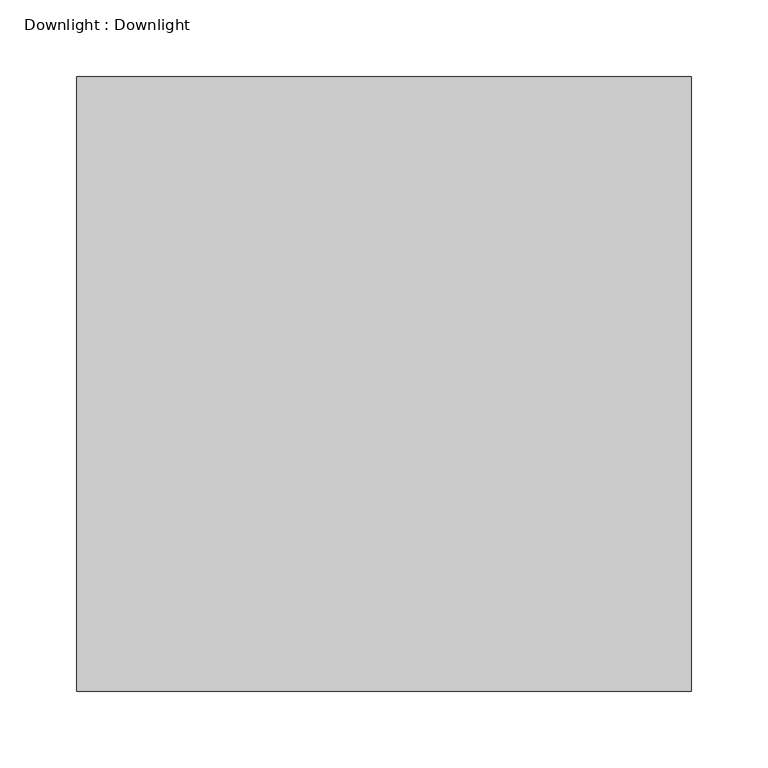
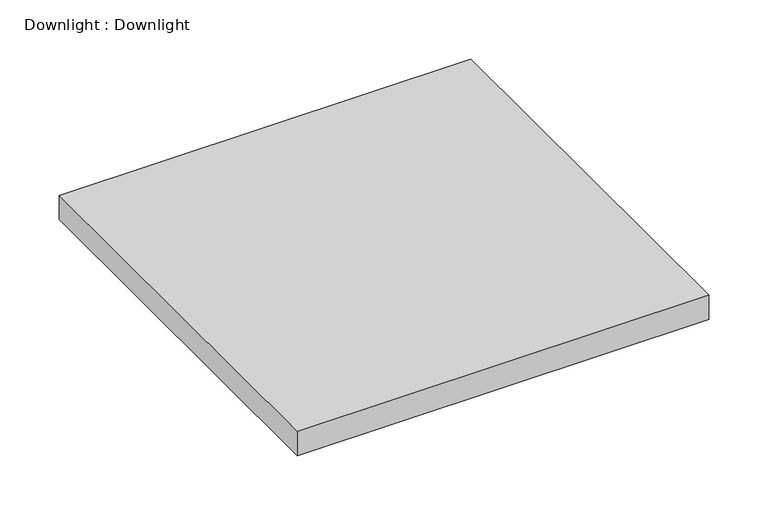
"""IFC4 building model written with IfcOpenShell, lengths in millimetres: light fixture geometry, Downlight : Downlight."""

from ifc_helpers import new_model, si_unit, frame, origin, place, context, project, spatial, polyline, outline, extrude, source, transform, mapped, element, save


def downlight_downlight_20077eaa(model_context):
    return source(origin(), model_context, "Body", "SweptSolid", [
        extrude(outline(polyline([(200.0, -200.0), (-200.0, -200.0), (-200.0, 200.0), (200.0, 200.0), (200.0, -200.0)])), frame((0.0, 0.0, -4.6872227), z_axis=(0.0, 0.0, 1.0), x_axis=(1.0, 0.0, 0.0)), (0.0, 0.0, 1.0), 24.9370919),
    ])


if __name__ == "__main__":
    model = new_model("IFC4")
    model_context = context("Model", 3, world=origin())
    ifc_project = project(units=[si_unit("LENGTHUNIT", "METRE", prefix="MILLI")], contexts=[model_context])
    site = spatial("IfcSite", under=ifc_project)
    building = spatial("IfcBuilding", under=site)
    placement = place(None, origin())
    downlight_downlight_shape = downlight_downlight_20077eaa(model_context)
    element("IfcLightFixture", 1, ObjectType="Downlight : Downlight", at=placement, inside=building, context=model_context, shape_type="MappedRepresentation", body=[
        mapped(downlight_downlight_shape, transform((0.0, 0.0, 0.0), x_axis=(1.0, 0.0, 0.0), y_axis=(0.0, 1.0, 0.0), z_axis=(0.0, 0.0, 1.0))),
    ])
    save(model, "model.ifc")

# Revit data of these elements
# Type "Downlight : Downlight"
#   Default Elevation = 0
